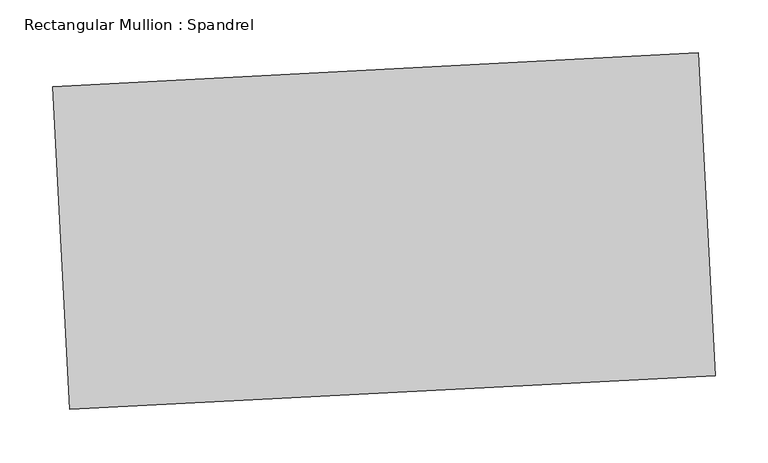
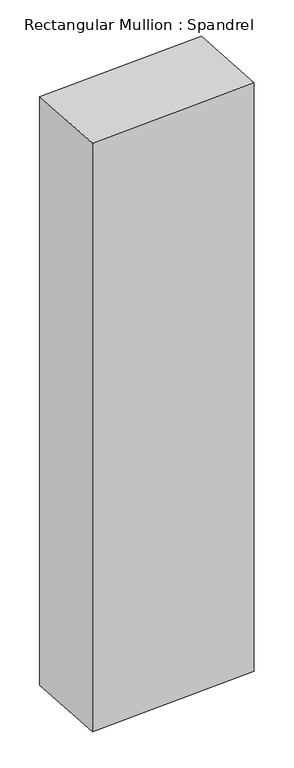
"""IFC4 building model written with IfcOpenShell, lengths in millimetres: member geometry, Rectangular Mullion : Spandrel."""

from ifc_helpers import new_model, si_unit, frame, origin, place, context, project, spatial, polyline, outline, extrude, source, transform, mapped, element, save


def rectangular_mullion_spandrel_372107e3(model_context):
    return source(origin(), model_context, "Body", "SweptSolid", [
        extrude(outline(polyline([(-617.1582819, 136.2391416), (-8.3937175, 168.1431406), (7.5582819, -136.2391416), (-601.2062825, -168.1431406), (-617.1582819, 136.2391416)])), frame((0.0, 0.0, -2268.2609739), z_axis=(0.0, 0.0, 1.0), x_axis=(1.0, 0.0, 0.0)), (0.0, 0.0, 1.0), 2268.2609739),
    ])


if __name__ == "__main__":
    model = new_model("IFC4")
    model_context = context("Model", 3, world=origin())
    ifc_project = project(units=[si_unit("LENGTHUNIT", "METRE", prefix="MILLI")], contexts=[model_context])
    site = spatial("IfcSite", under=ifc_project)
    building = spatial("IfcBuilding", under=site)
    placement = place(None, origin())
    rectangular_mullion_spandrel_shape = rectangular_mullion_spandrel_372107e3(model_context)
    element("IfcMember", 1, ObjectType="Rectangular Mullion : Spandrel", at=placement, inside=building, context=model_context, shape_type="MappedRepresentation", body=[
        mapped(rectangular_mullion_spandrel_shape, transform((0.0, 0.0, 0.0), x_axis=(1.0, 0.0, 0.0), y_axis=(0.0, 1.0, 0.0), z_axis=(0.0, 0.0, 1.0))),
    ])
    save(model, "model.ifc")

# Revit data of these elements
# Type "Rectangular Mullion : Spandrel"
#   built-in parameter 1007304 = 1 (stored number, unit not read)
#   built-in parameter 1007301 = 1 (stored number, unit not read)
#   built-in parameter 1007300 = 1 (stored number, unit not read)
# Element 1 (IfcMember, "Rectangular Mullion : Spandrel")
#   Materials on its faces: "Aluminum"
# Materials
#   "Aluminum": class "Metal", colour RGB 247 247 247, transparency 0, Description = "Aluminum 6061", Cost = 0
